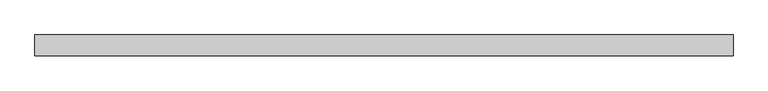
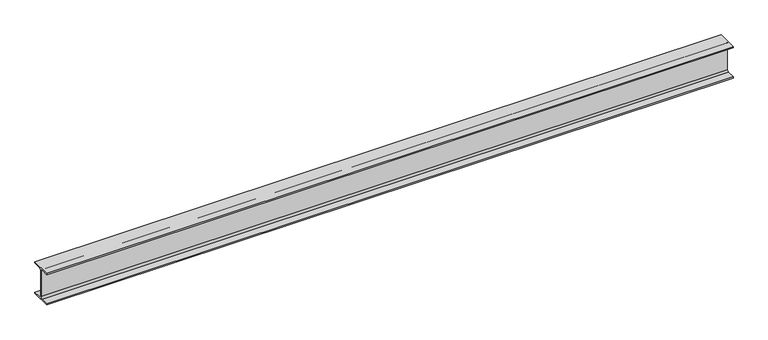
"""IFC4 building model written with IfcOpenShell, lengths in millimetres: beam geometry, 0912_Steel Framing_H-KSD3502 : H_SB_ASB_H-488x300x11x18."""

from ifc_helpers import new_model, si_unit, point, frame, frame_2d, origin, place, context, project, spatial, polyline, circle_curve, trimmed, segment, composite_curve, outline, extrude, source, transform, mapped, element, save


def beam_d932ca8a(model_context):
    return source(origin(), model_context, "Body", "SweptSolid", [
        extrude(outline(composite_curve([segment(polyline([(150.0, -226.0), (150.0, -244.0), (-150.0, -244.0), (-150.0, -226.0), (-31.5, -226.0)]), True, "CONTINUOUS"), segment(trimmed(circle_curve(frame_2d((-31.5, -200.0)), 26.0), [point((-31.5, -226.0))], [point((-5.5, -200.0))], True, "CARTESIAN"), True, "CONTINUOUS"), segment(polyline([(-5.5, -200.0), (-5.5, 200.0)]), True, "CONTINUOUS"), segment(trimmed(circle_curve(frame_2d((-31.5, 200.0)), 26.0), [point((-5.5, 200.0))], [point((-31.5, 226.0))], True, "CARTESIAN"), True, "CONTINUOUS"), segment(polyline([(-31.5, 226.0), (-150.0, 226.0), (-150.0, 244.0), (150.0, 244.0), (150.0, 226.0), (31.5, 226.0)]), True, "CONTINUOUS"), segment(trimmed(circle_curve(frame_2d((31.5, 200.0)), 26.0), [point((31.5, 226.0))], [point((5.5, 200.0))], True, "CARTESIAN"), True, "CONTINUOUS"), segment(polyline([(5.5, 200.0), (5.5, -200.0)]), True, "CONTINUOUS"), segment(trimmed(circle_curve(frame_2d((31.5, -200.0)), 26.0), [point((5.5, -200.0))], [point((31.5, -226.0))], True, "CARTESIAN"), True, "CONTINUOUS"), segment(polyline([(31.5, -226.0), (150.0, -226.0)]), True, "CONTINUOUS")], self_intersect=False)), frame((-5029.8, 0.0, 0.0), z_axis=(1.0, 0.0, 0.0), x_axis=(0.0, 1.0, 0.0)), (0.0, 0.0, 1.0), 10059.6),
    ])


if __name__ == "__main__":
    model = new_model("IFC4")
    model_context = context("Model", 3, world=origin())
    ifc_project = project(units=[si_unit("LENGTHUNIT", "METRE", prefix="MILLI")], contexts=[model_context])
    site = spatial("IfcSite", under=ifc_project)
    building = spatial("IfcBuilding", under=site)
    placement = place(None, origin())
    beam_shape = beam_d932ca8a(model_context)
    element("IfcBeam", 1, ObjectType="0912_Steel Framing_H-KSD3502 : H_SB_ASB_H-488x300x11x18", at=placement, inside=building, context=model_context, shape_type="MappedRepresentation", body=[
        mapped(beam_shape, transform((0.0, 0.0, 0.0), x_axis=(1.0, 0.0, 0.0), y_axis=(0.0, 1.0, 0.0), z_axis=(0.0, 0.0, 1.0))),
    ])
    save(model, "model.ifc")

# Revit data of these elements
# Type "0912_Steel Framing_H-KSD3502 : H_SB_ASB_H-488x300x11x18"
#   H_WM Code_1 = "S01AA001-00001 | Main Steel Structure Fabrication Work | Shelter/Building | Heavy Steel - Standard (Weight≥90KG/M) | Material: (   )"
#   H_WM Code_2 = "S03AA027-00001 | Main Steel Structure Erection Work | Shelter/Building | Heavy Steel (Weight≥90KG/M) | Material: (   )"
#   H_WM Code_3 = "S01AA010-00001 | Main Steel Structure Fabrication Work | Shelter/Building | Steel Painting/Coating | for Non-Fireproofed Steel Surface, Surface Preparation, Primer, Second & Final Coat | Material: (   )"
#   H_Q'ty Cal Type Tag = "SB-Q2"
#   Width = 30.0 cm
#   Web Thickness = 1.1 cm
#   Web Fillet = 2.6 cm
#   Warping Constant = 4470000.0 cm⁶
#   W = 0
#   Torsional Moment of Inertia = 137.492 cm⁴
#   Section Area = 163.5 cm²
#   Plastic Modulus weak axis = 830.0 cm³
#   Plastic Modulus strong axis = 3230.0 cm³
#   Perimeter = 2.11 m²/m
#   Nominal Weight = 128.00 kgf/m
#   Moment of Inertia weak axis = 8110.00 cm⁴
#   Moment of Inertia strong axis = 71000.00 cm⁴
#   Height = 48.8 cm
#   Flange Thickness = 1.8 cm
#   Elastic Modulus weak axis = 541.0 cm³
#   Elastic Modulus strong axis = 2910.0 cm³
#   Centroid Vertical = 24.4 cm
#   Centroid Horizontal = 15.0 cm
#   Ix = 710000000
#   Length [instance default] = 1.5240 m
#   Zx = 3230000
#   b = 0.3000 m
#   h = 0.4880 m
#   r = 0.0260 m
#   s = 0.0110 m
#   t = 0.0180 m
#   A = 0.01635 m²
#   Structural Material [instance default] = Steel, 45-345
#   Assembly Code = ""
# Element 1 (IfcBeam, "0912_Steel Framing_H-KSD3502 : H_SB_ASB_H-488x300x11x18")
#   Structural Material = none
# Materials
#   "Steel, 45-345": class "Metal", colour RGB 189 187 185, transparency 0, Description = "Steel 345 MPa", Cost = 0
